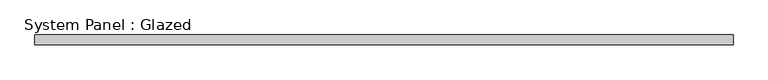
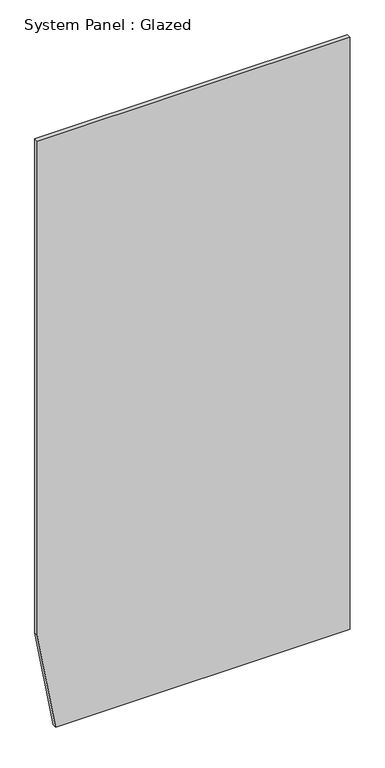
"""IFC4 building model written with IfcOpenShell, lengths in millimetres: plate geometry, System Panel : Glazed."""

from ifc_helpers import new_model, si_unit, frame, origin, place, context, project, spatial, polyline, outline, extrude, source, transform, mapped, element, save


def system_panel_glazed_866ab655(model_context):
    return source(origin(), model_context, "Body", "SweptSolid", [
        extrude(outline(polyline([(0.0, -808.3993064), (0.0, 914.4), (3657.6, 914.4), (3657.6, -914.4), (603.4561394, -914.4), (0.0, -808.3993064)])), frame((0.0, -44.45, 0.0), z_axis=(0.0, 1.0, 0.0), x_axis=(0.0, 0.0, 1.0)), (0.0, 0.0, 1.0), 25.4),
    ])


if __name__ == "__main__":
    model = new_model("IFC4")
    model_context = context("Model", 3, world=origin())
    ifc_project = project(units=[si_unit("LENGTHUNIT", "METRE", prefix="MILLI")], contexts=[model_context])
    site = spatial("IfcSite", under=ifc_project)
    building = spatial("IfcBuilding", under=site)
    placement = place(None, origin())
    system_panel_glazed_shape = system_panel_glazed_866ab655(model_context)
    element("IfcPlate", 1, ObjectType="System Panel : Glazed", at=placement, inside=building, context=model_context, shape_type="MappedRepresentation", body=[
        mapped(system_panel_glazed_shape, transform((0.0, 0.0, 0.0), x_axis=(1.0, 0.0, 0.0), y_axis=(0.0, 1.0, 0.0), z_axis=(0.0, 0.0, 1.0))),
    ])
    save(model, "model.ifc")

# Revit data of these elements
# Type "System Panel : Glazed"
#   Construction Type Id = "GSP4R"
#   Analytic Construction = "1/8 in Pilkington single glazing"
#   Visual Light Transmittance = 0.9
#   Solar Heat Gain Coefficient = 0.86
#   Heat Transfer Coefficient (U) = 1.18115 BTU/(h·ft²·°F)
#   Define Thermal Properties by = 1
# Element 1 (IfcPlate, "System Panel : Glazed")
#   Materials on its faces: "Glass"
# Materials
#   "Glass": class "Glass", colour RGB 0 128 192, transparency 0.75, Description = "Soda Lime Glass", Cost = 0
